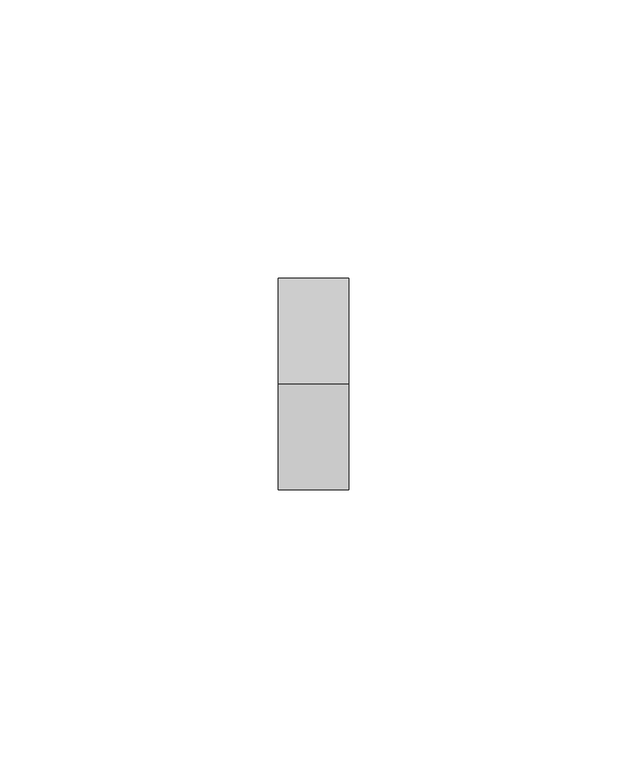
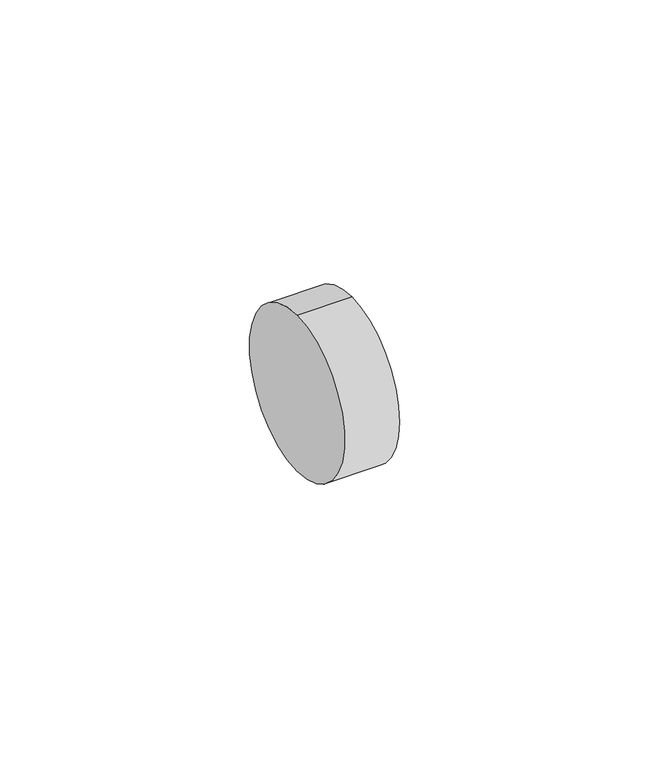
"""IFC4 building model written with IfcOpenShell, lengths in millimetres: proxy geometry, Bolt27:Bolt002:304721 : Bolt27:Bolt002:304721."""

from ifc_helpers import new_model, si_unit, point, frame, frame_2d, origin, place, context, project, spatial, circle_curve, trimmed, segment, composite_curve, outline, extrude, source, transform, mapped, element, save


def generic_models_6a9c452d(model_context):
    return source(origin(), model_context, "Body", "SweptSolid", [
        extrude(outline(composite_curve([segment(trimmed(circle_curve(frame_2d((2264.1630212, 40070.0545241)), 19.05), [point((2264.1630212, 40051.0045241))], [point((2264.1630212, 40089.1045241))], False, "CARTESIAN"), True, "CONTINUOUS"), segment(trimmed(circle_curve(frame_2d((2264.1630212, 40070.0545241)), 19.05), [point((2264.1630212, 40089.1045241))], [point((2264.1630212, 40051.0045241))], False, "CARTESIAN"), True, "CONTINUOUS")], self_intersect=False)), frame((15045.2731889, 0.0, 0.0), z_axis=(1.0, 0.0, 0.0), x_axis=(0.0, 1.0, 0.0)), (0.0, 0.0, 1.0), 12.7),
    ])


if __name__ == "__main__":
    model = new_model("IFC4")
    model_context = context("Model", 3, world=origin())
    ifc_project = project(units=[si_unit("LENGTHUNIT", "METRE", prefix="MILLI")], contexts=[model_context])
    site = spatial("IfcSite", under=ifc_project)
    building = spatial("IfcBuilding", under=site)
    placement = place(None, origin())
    generic_models_shape = generic_models_6a9c452d(model_context)
    element("IfcBuildingElementProxy", 1, Name="Bolt27:Bolt002:304721 : Bolt27:Bolt002:304721", ObjectType="Bolt27:Bolt002:304721 : Bolt27:Bolt002:304721", at=placement, inside=building, context=model_context, shape_type="MappedRepresentation", body=[
        mapped(generic_models_shape, transform((0.0, 0.0, 0.0), x_axis=(1.0, 0.0, 0.0), y_axis=(0.0, 1.0, 0.0), z_axis=(0.0, 0.0, 1.0))),
    ])
    save(model, "model.ifc")

# Revit data of these elements
# Type "Bolt27:Bolt002:304721 : Bolt27:Bolt002:304721"
#   NameOverride = "Bolt27:Bolt002:304721"
#   ObjectTypeOverride = "Bolt27:Bolt002"
#   Reference = "Bolt002"
#   Category = "Generic Models"
#   Tag = "304721"
# Element 1 (IfcBuildingElementProxy, "Bolt27:Bolt002:304721 : Bolt27:Bolt002:304721")
#   Materials on its faces: "TUBE STEEL STRINGER WELDED TO ANCHORED STEEL PLATE - SEE STRUCT DWGS"
# Materials
#   "TUBE STEEL STRINGER WELDED TO ANCHORED STEEL PLATE - SEE STRUCT DWGS": class "Unassigned", colour RGB 128 128 128, transparency 0, Cost = 0
